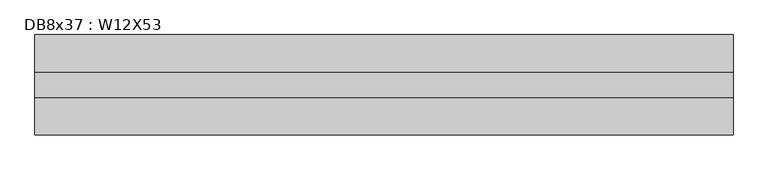
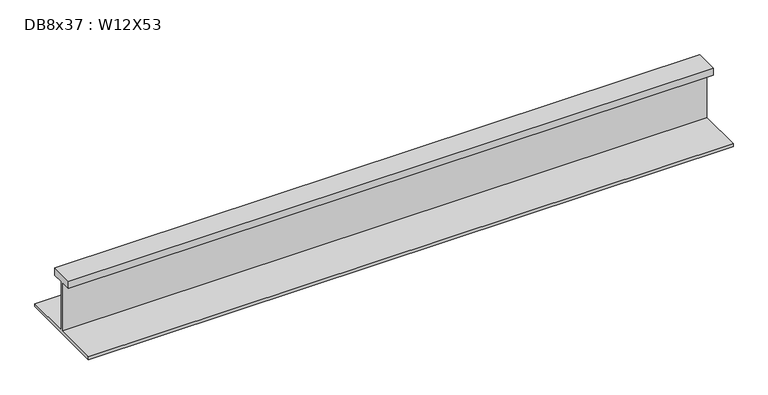
"""IFC4 building model written with IfcOpenShell, lengths in millimetres: beam geometry, DB8x37 : W12X53."""

from ifc_helpers import new_model, si_unit, frame, origin, place, context, project, spatial, polyline, outline, extrude, source, transform, mapped, element, save


def db8x37_w12x53_d1be734d(model_context):
    return source(origin(), model_context, "Body", "SweptSolid", [
        extrude(outline(polyline([(38.1, 145.415), (38.1, 120.015), (2.921, 120.015), (2.921, -48.4505), (152.4, -48.4505), (152.4, -58.1025), (-152.4, -58.1025), (-152.4, -48.4505), (-2.921, -48.4505), (-2.921, 120.015), (-38.1, 120.015), (-38.1, 145.415), (38.1, 145.415)])), frame((-1019.9407413, 0.0, 0.0), z_axis=(1.0, 0.0, 0.0), x_axis=(0.0, 1.0, 0.0)), (0.0, 0.0, 1.0), 2119.1566634),
    ])


if __name__ == "__main__":
    model = new_model("IFC4")
    model_context = context("Model", 3, world=origin())
    ifc_project = project(units=[si_unit("LENGTHUNIT", "METRE", prefix="MILLI")], contexts=[model_context])
    site = spatial("IfcSite", under=ifc_project)
    building = spatial("IfcBuilding", under=site)
    placement = place(None, origin())
    db8x37_w12x53_shape = db8x37_w12x53_d1be734d(model_context)
    element("IfcBeam", 1, ObjectType="DB8x37 : W12X53", at=placement, inside=building, context=model_context, shape_type="MappedRepresentation", body=[
        mapped(db8x37_w12x53_shape, transform((0.0, 0.0, 0.0), x_axis=(1.0, 0.0, 0.0), y_axis=(0.0, 1.0, 0.0), z_axis=(0.0, 0.0, 1.0))),
    ])
    save(model, "model.ifc")

# Revit data of these elements
# Type "DB8x37 : W12X53"
#   Assembly Code = "B10"
#   W = 53
#   Length [instance default] = 5' - 0"
#   bf = 0' - 10"
#   d = 1' - 0.1"
#   k = 0' - 1 3/8"
#   k2 = 0' - 0.8"
#   tf = 0' - 0.575"
#   tw = 0' - 0.345"
#   A = 0.108333 SF
#   Structural Material [instance default] = Steel ASTM A992
# Element 1 (IfcBeam, "DB8x37 : W12X53")
#   Materials on its faces: "Steel ASTM A992"
# Materials
#   "Steel ASTM A992": class "Metal", colour RGB 199 199 199, transparency 0, Description = "Structural steel 50ksi", Cost = 0
